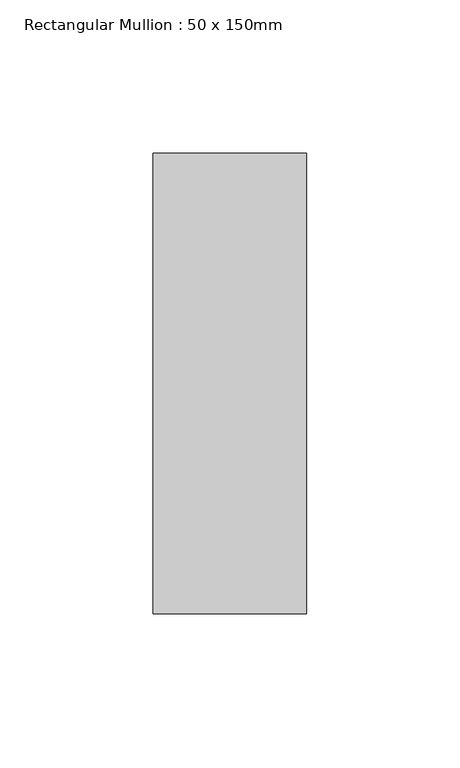
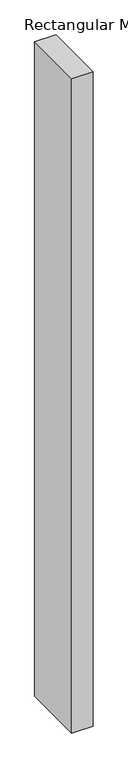
"""IFC4 building model written with IfcOpenShell, lengths in millimetres: member geometry, Rectangular Mullion : 50 x 150mm."""

from ifc_helpers import new_model, si_unit, frame, origin, place, context, project, spatial, polyline, outline, extrude, source, transform, mapped, element, save


def rectangular_mullion_50_x_150mm_f3f87aca(model_context):
    return source(origin(), model_context, "Body", "SweptSolid", [
        extrude(outline(polyline([(0.0, 75.0), (0.0, -75.0), (-50.0, -75.0), (-50.0, 75.0), (0.0, 75.0)])), frame((0.0, 0.0, -1620.0), z_axis=(0.0, 0.0, 1.0), x_axis=(1.0, 0.0, 0.0)), (0.0, 0.0, 1.0), 1620.0),
    ])


if __name__ == "__main__":
    model = new_model("IFC4")
    model_context = context("Model", 3, world=origin())
    ifc_project = project(units=[si_unit("LENGTHUNIT", "METRE", prefix="MILLI")], contexts=[model_context])
    site = spatial("IfcSite", under=ifc_project)
    building = spatial("IfcBuilding", under=site)
    placement = place(None, origin())
    rectangular_mullion_50_x_150mm_shape = rectangular_mullion_50_x_150mm_f3f87aca(model_context)
    element("IfcMember", 1, ObjectType="Rectangular Mullion : 50 x 150mm", at=placement, inside=building, context=model_context, shape_type="MappedRepresentation", body=[
        mapped(rectangular_mullion_50_x_150mm_shape, transform((0.0, 0.0, 0.0), x_axis=(1.0, 0.0, 0.0), y_axis=(0.0, 1.0, 0.0), z_axis=(0.0, 0.0, 1.0))),
    ])
    save(model, "model.ifc")

# Revit data of these elements
# Type "Rectangular Mullion : 50 x 150mm"
#   built-in parameter 1007304 = 0.492126 (stored number, unit not read)
#   built-in parameter 1007301 = 0.082021 (stored number, unit not read)
#   built-in parameter 1007300 = 0.082021 (stored number, unit not read)
# Element 1 (IfcMember, "Rectangular Mullion : 50 x 150mm")
#   Materials on its faces: "Metal - Aluminium"
# Materials
#   "Metal - Aluminium": class "Metal", colour RGB 247 247 247, transparency 0
